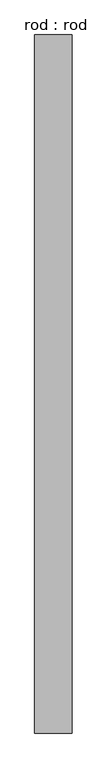
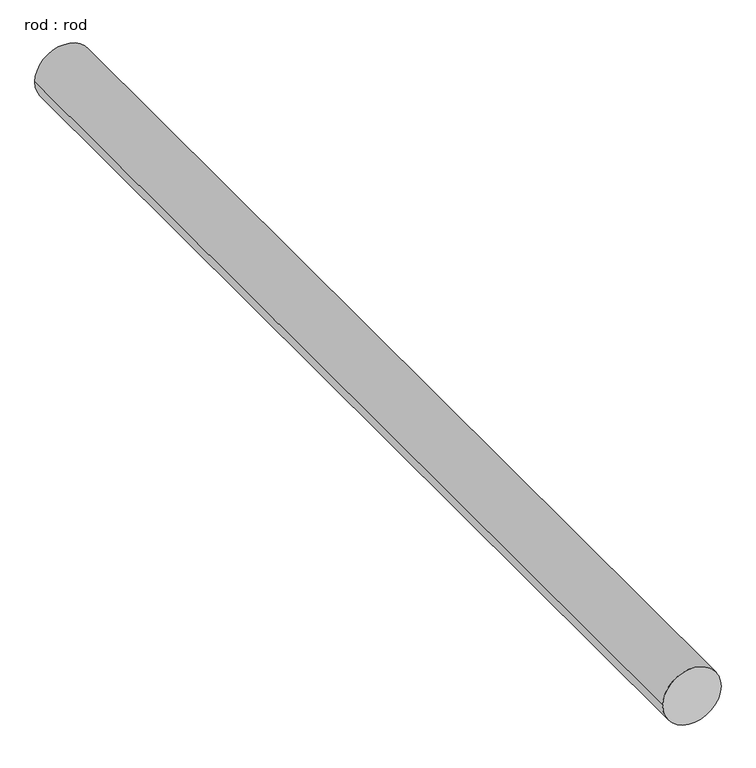
"""IFC4 building model written with IfcOpenShell, lengths in millimetres: proxy geometry, rod : rod."""

from ifc_helpers import new_model, si_unit, point, frame, frame_2d, origin, place, context, project, spatial, circle_curve, trimmed, segment, composite_curve, outline, extrude, source, transform, mapped, element, save


def rod_rod_309aab9d(model_context):
    return source(origin(), model_context, "Body", "SweptSolid", [
        extrude(outline(composite_curve([segment(trimmed(circle_curve(frame_2d((0.0108462, 0.0)), 200.0), [point((0.0108462, 200.0))], [point((0.0108462, -200.0))], False, "CARTESIAN"), True, "CONTINUOUS"), segment(trimmed(circle_curve(frame_2d((0.0108462, 0.0)), 200.0), [point((0.0108462, -200.0))], [point((0.0108462, 200.0))], False, "CARTESIAN"), True, "CONTINUOUS")], self_intersect=False)), frame((0.0, 365.9832189, 0.0), z_axis=(0.0, 1.0, 0.0), x_axis=(0.0, 0.0, 1.0)), (0.0, 0.0, 1.0), 7453.4907929),
    ])


if __name__ == "__main__":
    model = new_model("IFC4")
    model_context = context("Model", 3, world=origin())
    ifc_project = project(units=[si_unit("LENGTHUNIT", "METRE", prefix="MILLI")], contexts=[model_context])
    site = spatial("IfcSite", under=ifc_project)
    building = spatial("IfcBuilding", under=site)
    placement = place(None, origin())
    rod_rod_shape = rod_rod_309aab9d(model_context)
    element("IfcBuildingElementProxy", 1, Name="rod : rod", ObjectType="rod : rod", at=placement, inside=building, context=model_context, shape_type="MappedRepresentation", body=[
        mapped(rod_rod_shape, transform((0.0, 0.0, 0.0), x_axis=(1.0, 0.0, 0.0), y_axis=(0.0, 1.0, 0.0), z_axis=(0.0, 0.0, 1.0))),
    ])
    save(model, "model.ifc")

# Revit data of these elements
# Type "rod : rod"
#   Default Elevation = 0
